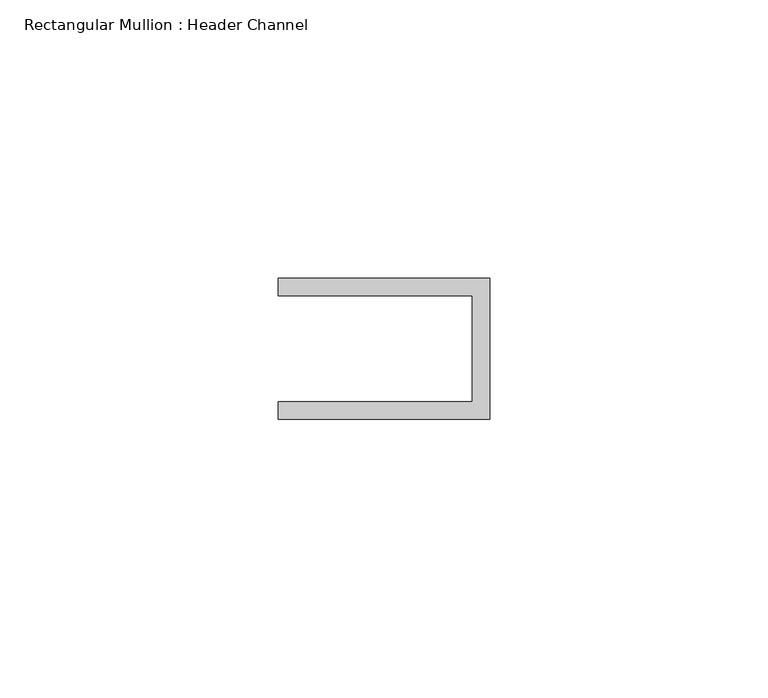
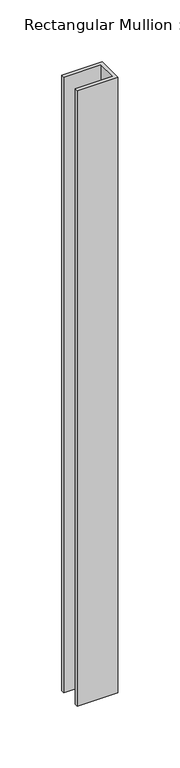
"""IFC4 building model written with IfcOpenShell, lengths in millimetres: member geometry, Rectangular Mullion : Header Channel."""

from ifc_helpers import new_model, si_unit, frame, origin, place, context, project, spatial, polyline, outline, extrude, source, transform, mapped, element, save


def rectangular_mullion_header_channel_868cf06b(model_context):
    return source(origin(), model_context, "Body", "SweptSolid", [
        extrude(outline(polyline([(0.0, -12.7), (-38.1, -12.7), (-38.1, -9.525), (-3.175, -9.525), (-3.175, 9.525), (-38.1, 9.525), (-38.1, 12.7), (0.0, 12.7), (0.0, -12.7)])), frame((0.0, 0.0, -609.6), z_axis=(0.0, 0.0, 1.0), x_axis=(1.0, 0.0, 0.0)), (0.0, 0.0, 1.0), 609.6),
    ])


if __name__ == "__main__":
    model = new_model("IFC4")
    model_context = context("Model", 3, world=origin())
    ifc_project = project(units=[si_unit("LENGTHUNIT", "METRE", prefix="MILLI")], contexts=[model_context])
    site = spatial("IfcSite", under=ifc_project)
    building = spatial("IfcBuilding", under=site)
    placement = place(None, origin())
    rectangular_mullion_header_channel_shape = rectangular_mullion_header_channel_868cf06b(model_context)
    element("IfcMember", 1, ObjectType="Rectangular Mullion : Header Channel", at=placement, inside=building, context=model_context, shape_type="MappedRepresentation", body=[
        mapped(rectangular_mullion_header_channel_shape, transform((0.0, 0.0, 0.0), x_axis=(1.0, 0.0, 0.0), y_axis=(0.0, 1.0, 0.0), z_axis=(0.0, 0.0, 1.0))),
    ])
    save(model, "model.ifc")

# Revit data of these elements
# Type "Rectangular Mullion : Header Channel"
#   built-in parameter 1007322 = 0.0833333 (stored number, unit not read)
#   built-in parameter 1007321 = -0.03125 (stored number, unit not read)
#   built-in parameter 1007320 = 0.0416667 (stored number, unit not read)
# Element 1 (IfcMember, "Rectangular Mullion : Header Channel")
#   Materials on its faces: "ALUM"
# Materials
#   "ALUM": class "Generic", colour RGB 157 157 157, transparency 0, Cost = 0
